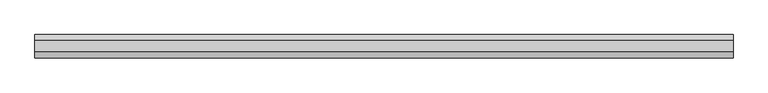
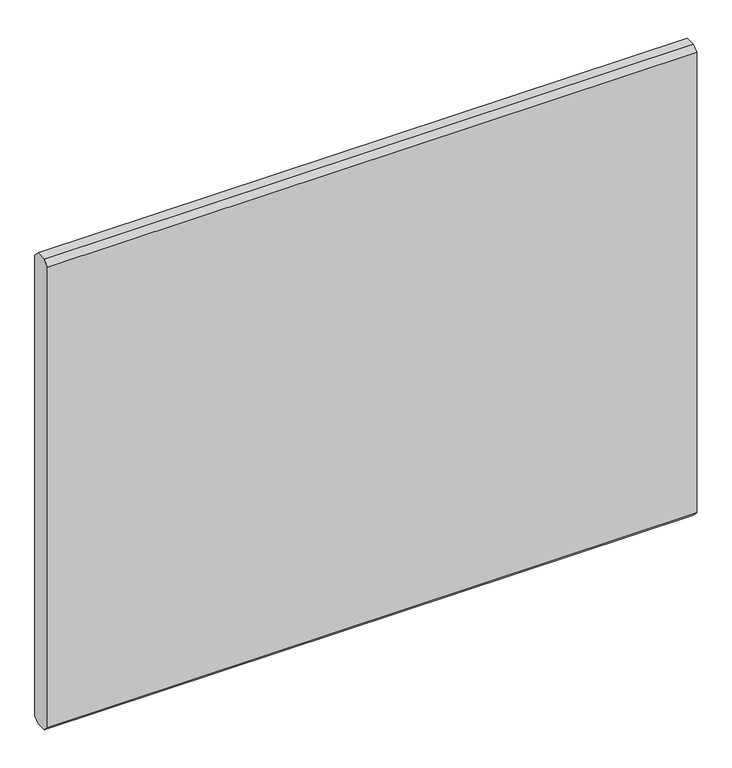
"""IFC4 building model written with IfcOpenShell, lengths in millimetres: proxy geometry, .RIPA : RIPA."""

from ifc_helpers import new_model, si_unit, frame, origin, place, context, project, spatial, polyline, outline, extrude, source, transform, mapped, element, save


def generic_models_02b59547(model_context):
    return source(origin(), model_context, "Body", "SweptSolid", [
        extrude(outline(polyline([(-12.5, 1150.0), (12.5, 1150.0), (25.0, 1137.5), (25.0, 12.5), (12.5, 0.0), (-12.5, 0.0), (-25.0, 12.5), (-25.0, 1137.5), (-12.5, 1150.0)])), frame((-750.0, 0.0, 0.0), z_axis=(1.0, 0.0, 0.0), x_axis=(0.0, 1.0, 0.0)), (0.0, 0.0, 1.0), 1500.0),
    ])


if __name__ == "__main__":
    model = new_model("IFC4")
    model_context = context("Model", 3, world=origin())
    ifc_project = project(units=[si_unit("LENGTHUNIT", "METRE", prefix="MILLI")], contexts=[model_context])
    site = spatial("IfcSite", under=ifc_project)
    building = spatial("IfcBuilding", under=site)
    placement = place(None, origin())
    generic_models_shape = generic_models_02b59547(model_context)
    element("IfcBuildingElementProxy", 1, Name=".RIPA : RIPA", ObjectType=".RIPA : RIPA", at=placement, inside=building, context=model_context, shape_type="MappedRepresentation", body=[
        mapped(generic_models_shape, transform((0.0, 0.0, 0.0), x_axis=(1.0, 0.0, 0.0), y_axis=(0.0, 1.0, 0.0), z_axis=(0.0, 0.0, 1.0))),
    ])
    save(model, "model.ifc")

# Revit data of these elements
# Type ".RIPA : RIPA"
#   Ripa_largura [instance default] = 0.30 m
#   Ripa_espessura [instance default] = 0.025 m
#   Ripa_comprimento [instance default] = 0.80 m
#   Ripa_chanfo [instance default] = 0.00625 m
#   Ripa_material [instance default] = none
# Element 1 (IfcBuildingElementProxy, ".RIPA : RIPA")
#   Ripa_largura = 1.15 m
#   Ripa_espessura = 0.05 m
#   Ripa_comprimento = 1.50 m
#   Ripa_chanfo = 0.0125 m
#   Ripa_material = .MADEIRA_CEREJEIRA CLARO
#   Materials on its faces: ".MADEIRA_CEREJEIRA CLARO"
# Materials
#   ".MADEIRA_CEREJEIRA CLARO": class ".CC_MADEIRA REVEST.", colour RGB 233 182 144, transparency 0, Cost = 0
